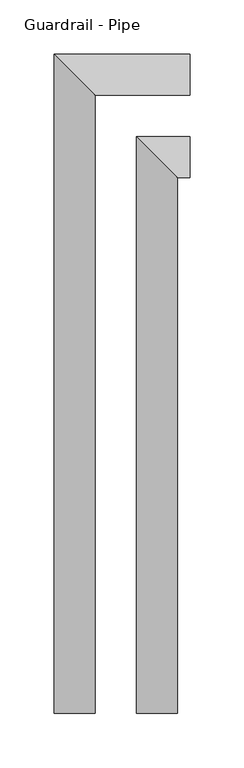
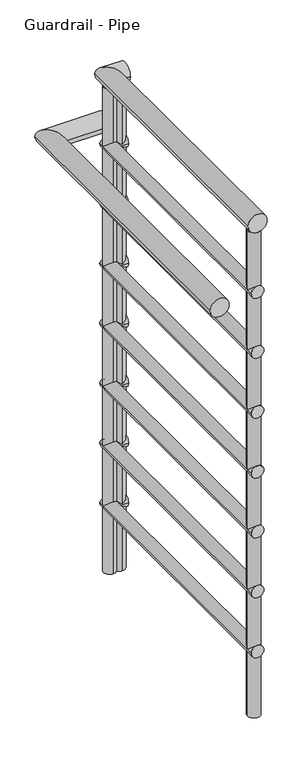
"""IFC4 building model written with IfcOpenShell, lengths in millimetres: railing geometry, Guardrail - Pipe."""

import ifcopenshell
import ifcopenshell.guid

model = None  # the IFC model being written
_history = None  # IfcOwnerHistory: only IFC2X3 demands one
_inside = {}  # id of a spatial element -> (the spatial element, [elements in it])
_under = {}  # id of a project, library or spatial element -> (it, [spatial elements below it])
_declared = {}  # id of a project -> (the project, [libraries it declares])
_typed = {}  # id of a type object -> (the type object, [elements of that type])
_made_of = {}  # id of a material, layer set ... -> (it, [elements and type objects made of it])


def new_model(schema):
    """Start an empty IFC model of exactly this schema.

    Asked for "IFC4X3", IfcOpenShell would pick the latest addendum, in which some entities
    have other attributes; the version numbers below select the first issue.
    IFC2X3 requires an IfcOwnerHistory on every rooted entity: one is made here for all.
    """
    global model, _history
    if schema == "IFC4X3":
        model = ifcopenshell.file(schema_version=(4, 3, 0, 0))
    else:
        model = ifcopenshell.file(schema=schema)
    _inside.clear()
    _under.clear()
    _declared.clear()
    _typed.clear()
    _made_of.clear()
    _history = None
    if model.schema == "IFC2X3":
        org = make("IfcOrganization", Name="unknown")
        user = make(
            "IfcPersonAndOrganization",
            ThePerson=make("IfcPerson", FamilyName="unknown"),
            TheOrganization=org,
        )
        app = make(
            "IfcApplication",
            ApplicationDeveloper=org,
            Version="unknown",
            ApplicationFullName="unknown",
            ApplicationIdentifier="unknown",
        )
        _history = make(
            "IfcOwnerHistory",
            OwningUser=user,
            OwningApplication=app,
            ChangeAction="ADDED",
            CreationDate=0,
        )
    return model


def make(cls, **values):
    """One entity of the class cls with the attributes given. An attribute that is None is left unset."""
    return model.create_entity(
        cls, **{name: value for name, value in values.items() if value is not None}
    )


def rooted(cls, **values):
    """An entity with a GlobalId (a new one), such as an element, a storey or a relation."""
    return make(cls, GlobalId=ifcopenshell.guid.new(), OwnerHistory=_history, **values)


def si_unit(unit_type, name, prefix=None):
    """IfcSIUnit, for example si_unit("LENGTHUNIT", "METRE", prefix="MILLI")."""
    return make("IfcSIUnit", UnitType=unit_type, Prefix=prefix, Name=name)


def assignment(units):
    """IfcUnitAssignment: the units of a project."""
    return None if units is None else make("IfcUnitAssignment", Units=units)


def point(xyz):
    """IfcCartesianPoint."""
    return None if xyz is None else make("IfcCartesianPoint", Coordinates=xyz)


def direction(xyz):
    """IfcDirection."""
    return None if xyz is None else make("IfcDirection", DirectionRatios=xyz)


def frame(location, z_axis=None, x_axis=None):
    """IfcAxis2Placement3D, a coordinate frame: its origin and axes. An axis left out is left unset."""
    return make(
        "IfcAxis2Placement3D",
        Location=point(location),
        Axis=direction(z_axis),
        RefDirection=direction(x_axis),
    )


def frame_2d(location, x_axis=None):
    """IfcAxis2Placement2D, a coordinate frame in the plane: its origin and x axis."""
    return make(
        "IfcAxis2Placement2D", Location=point(location), RefDirection=direction(x_axis)
    )


def origin():
    """The frame at (0, 0, 0) with its axes left unset."""
    return frame((0.0, 0.0, 0.0))


def place(relative_to, where):
    """IfcLocalPlacement: puts the frame where relative to a parent placement (None: the world)."""
    return make(
        "IfcLocalPlacement", PlacementRelTo=relative_to, RelativePlacement=where
    )


def context(
    kind, dimensions, precision=None, world=None, true_north=None, identifier=None
):
    """IfcGeometricRepresentationContext, for example the 3D "Model" context."""
    return make(
        "IfcGeometricRepresentationContext",
        ContextIdentifier=identifier,
        ContextType=kind,
        CoordinateSpaceDimension=dimensions,
        Precision=precision,
        WorldCoordinateSystem=world,
        TrueNorth=true_north,
    )


def project(units=None, contexts=None):
    """IfcProject with its units and contexts."""
    return rooted(
        "IfcProject",
        Name="project",
        RepresentationContexts=contexts,
        UnitsInContext=assignment(units),
    )


def spatial(cls, under=None, at=None, **own):
    """A site, building, storey or space (cls), placed at a placement, below another one or the project."""
    s = rooted(cls, ObjectPlacement=at, **own)
    if under is not None:
        _under.setdefault(under.id(), (under, []))[1].append(s)
    return s


def circle_curve(where, radius):
    """IfcCircle in the frame where."""
    return make("IfcCircle", Position=where, Radius=radius)


def ellipse_curve(where, semi_axis1, semi_axis2):
    """IfcEllipse in the frame where."""
    return make(
        "IfcEllipse", Position=where, SemiAxis1=semi_axis1, SemiAxis2=semi_axis2
    )


def trimmed(basis, trim1, trim2, sense, master):
    """IfcTrimmedCurve: the piece of a basis curve between two trims."""
    return make(
        "IfcTrimmedCurve",
        BasisCurve=basis,
        Trim1=trim1,
        Trim2=trim2,
        SenseAgreement=sense,
        MasterRepresentation=master,
    )


def segment(curve, same_sense, transition):
    """IfcCompositeCurveSegment."""
    return make(
        "IfcCompositeCurveSegment",
        Transition=transition,
        SameSense=same_sense,
        ParentCurve=curve,
    )


def composite_curve(segments, self_intersect=None):
    """IfcCompositeCurve: segments joined end to end."""
    return make("IfcCompositeCurve", Segments=segments, SelfIntersect=self_intersect)


def outline(outer, holes=None, kind="AREA"):
    """IfcArbitraryClosedProfileDef: a profile drawn as a closed curve; with holes, ...WithVoids."""
    if holes is None:
        return make("IfcArbitraryClosedProfileDef", ProfileType=kind, OuterCurve=outer)
    return make(
        "IfcArbitraryProfileDefWithVoids",
        ProfileType=kind,
        OuterCurve=outer,
        InnerCurves=holes,
    )


def extrude(swept, where, along, depth):
    """IfcExtrudedAreaSolid: the profile swept, set in the frame where, extruded along a direction by depth."""
    return make(
        "IfcExtrudedAreaSolid",
        SweptArea=swept,
        Position=where,
        ExtrudedDirection=direction(along),
        Depth=depth,
    )


def shape(context_of_items, identifier, shape_type, items):
    """IfcShapeRepresentation: the items that make up one representation, for example the "Body"."""
    return make(
        "IfcShapeRepresentation",
        ContextOfItems=context_of_items,
        RepresentationIdentifier=identifier,
        RepresentationType=shape_type,
        Items=items,
    )


def source(mapping_origin, context_of_items, identifier, shape_type, items):
    """IfcRepresentationMap: a shape defined once, which mapped items show again and again."""
    return make(
        "IfcRepresentationMap",
        MappingOrigin=mapping_origin,
        MappedRepresentation=shape(context_of_items, identifier, shape_type, items),
    )


def transform(
    local_origin,
    x_axis=None,
    y_axis=None,
    z_axis=None,
    scale=None,
    scale2=None,
    scale3=None,
    uniform=True,
):
    """IfcCartesianTransformationOperator3D, or its non-uniform kind. x_axis, y_axis, z_axis: its Axis1, 2, 3."""
    if uniform:
        return make(
            "IfcCartesianTransformationOperator3D",
            Axis1=direction(x_axis),
            Axis2=direction(y_axis),
            LocalOrigin=point(local_origin),
            Scale=scale,
            Axis3=direction(z_axis),
        )
    return make(
        "IfcCartesianTransformationOperator3DnonUniform",
        Axis1=direction(x_axis),
        Axis2=direction(y_axis),
        LocalOrigin=point(local_origin),
        Scale=scale,
        Axis3=direction(z_axis),
        Scale2=scale2,
        Scale3=scale3,
    )


def mapped(mapping_source, mapping_target):
    """IfcMappedItem: shows the shape of a source again, moved by a transform."""
    return make(
        "IfcMappedItem", MappingSource=mapping_source, MappingTarget=mapping_target
    )


def made_of(thing, what):
    """Note that an element or type object is made of a material, layer set ...; save() writes the relation."""
    if what is not None:
        _made_of.setdefault(what.id(), (what, []))[1].append(thing)
    return thing


def element(
    cls,
    number,
    at=None,
    inside=None,
    cuts=None,
    type_object=None,
    material=None,
    context=None,
    identifier="Body",
    shape_type=None,
    held_by="IfcProductDefinitionShape",
    body=None,
    shapes=None,
    **own,
):
    """One element of the class cls, such as IfcWall. Its Tag is "e" and its number.

    at: its placement. inside: the storey or other place that contains it. cuts: it is an
    opening in that element (IfcRelVoidsElement). A single representation is given by context,
    identifier, shape_type and body (its items); several are given by shapes. held_by: the class
    of the entity that holds the representations. save() writes the other relations.
    """
    e = rooted(cls, Tag="e%d" % number, ObjectPlacement=at, **own)
    if body is not None:
        shapes = [shape(context, identifier, shape_type, body)]
    if shapes is not None:
        e.Representation = make(held_by, Representations=shapes)
    if inside is not None:
        _inside.setdefault(inside.id(), (inside, []))[1].append(e)
    if cuts is not None:
        rooted(
            "IfcRelVoidsElement", RelatingBuildingElement=cuts, RelatedOpeningElement=e
        )
    if type_object is not None:
        _typed.setdefault(type_object.id(), (type_object, []))[1].append(e)
    return made_of(e, material)


def aggregate(whole, parts):
    """IfcRelAggregates: a whole, such as a stair, and the parts it consists of."""
    return rooted("IfcRelAggregates", RelatingObject=whole, RelatedObjects=parts)


def save(model, path):
    """Write the relations noted so far, then the file.

    IfcRelAggregates (storeys below a building ...), IfcRelContainedInSpatialStructure (elements
    in a storey), IfcRelDefinesByType, IfcRelAssociatesMaterial and IfcRelDeclares: one each for
    every whole, place, type object, material and project.
    """
    for whole, parts in _under.values():
        aggregate(whole, parts)
    for where, things in _inside.values():
        rooted(
            "IfcRelContainedInSpatialStructure",
            RelatedElements=things,
            RelatingStructure=where,
        )
    for kind, things in _typed.values():
        rooted("IfcRelDefinesByType", RelatedObjects=things, RelatingType=kind)
    for what, things in _made_of.values():
        rooted("IfcRelAssociatesMaterial", RelatedObjects=things, RelatingMaterial=what)
    for by, libraries in _declared.values():
        rooted("IfcRelDeclares", RelatingContext=by, RelatedDefinitions=libraries)
    model.write(path)


def plane_surface(at):
    """IfcPlane: the flat surface through the origin of the frame at, square to its z axis."""
    return make("IfcPlane", Position=at)


def cylinder_surface(at, radius):
    """IfcCylindricalSurface: all points at the distance radius from the z axis of the frame at."""
    return make("IfcCylindricalSurface", Position=at, Radius=radius)


def advanced_brep(points, edges, surfaces, faces):
    """IfcAdvancedBrep: a solid bounded by faces that lie on surfaces and meet in shared edges.

    An edge is (start, end): straight between two places in points (the first is 0);
    or (start, end, curve); or (start, end, curve, False) where it runs against its curve.
    A face is (place in surfaces, loops), or (place, loops, False) where it looks against
    its surface's normal. A loop lists edges by number (the first is 1), with a minus sign
    where the edge is run from its end to its start. The first loop is the outer one.
    """
    corners = [point(p) for p in points]
    vertices = [make("IfcVertexPoint", VertexGeometry=c) for c in corners]
    made = []
    for start, end, *more in edges:
        made.append(
            make(
                "IfcEdgeCurve",
                EdgeStart=vertices[start],
                EdgeEnd=vertices[end],
                EdgeGeometry=more[0] if more else make("IfcPolyline", Points=[corners[start], corners[end]]),
                SameSense=more[1] if len(more) > 1 else True,
            )
        )
    hull = []
    for where, loops, *sense in faces:
        bounds = []
        for j, loop in enumerate(loops):
            ring = [make("IfcOrientedEdge", EdgeElement=made[abs(k) - 1], Orientation=k > 0) for k in loop]
            bounds.append(
                make(
                    "IfcFaceOuterBound" if j == 0 else "IfcFaceBound",
                    Bound=make("IfcEdgeLoop", EdgeList=ring),
                    Orientation=True,
                )
            )
        hull.append(make("IfcAdvancedFace", Bounds=bounds, FaceSurface=surfaces[where], SameSense=sense[0] if sense else True))
    return make("IfcAdvancedBrep", Outer=make("IfcClosedShell", CfsFaces=hull))


def guardrail_pipe_cdf6dc9d(model_context):
    return source(origin(), model_context, "Body", "SolidModel", [
        advanced_brep(
        [(-10694.8293787, -5457.4797826, 4705.35), (-10656.7293787, -5457.4797826, 4705.35), (-10694.8293787, -4924.0797826, 4705.35), (-10656.7293787, -4962.1797826, 4705.35), (-10645.1029016, -4924.0797826, 4705.35), (-10645.1029016, -4962.1797826, 4705.35)],
        [
            (0, 1, circle_curve(frame((-10675.7793787, -5457.4797826, 4705.35), z_axis=(0.0, -1.0, 0.0), x_axis=(1.0, 0.0, 0.0)), 19.05)),
            (1, 0, circle_curve(frame((-10675.7793787, -5457.4797826, 4705.35), z_axis=(0.0, -1.0, 0.0), x_axis=(1.0, 0.0, 0.0)), 19.05)),
            (2, 3, ellipse_curve(frame((-10675.7793787, -4943.1297826, 4705.35), z_axis=(-0.7071067811865502, -0.7071067811865449, 0.0), x_axis=(-0.707106781186545, 0.70710678118655, 0.0)), 26.9407684, 19.05)),
            (3, 1),
            (0, 2),
            (3, 2, ellipse_curve(frame((-10675.7793787, -4943.1297826, 4705.35), z_axis=(-0.7071067811865502, -0.7071067811865449, 0.0), x_axis=(-0.707106781186545, 0.70710678118655, 0.0)), 26.9407684, 19.05)),
            (4, 5, circle_curve(frame((-10645.1029016, -4943.1297826, 4705.35), z_axis=(1.0, 0.0, 0.0), x_axis=(0.0, -1.0, 0.0)), 19.05)),
            (5, 4, circle_curve(frame((-10645.1029016, -4943.1297826, 4705.35), z_axis=(1.0, 0.0, 0.0), x_axis=(0.0, -1.0, 0.0)), 19.05)),
            (5, 3),
            (2, 4),
        ],
        [
            plane_surface(frame((-10675.7793787, -5457.4797826, 4724.4), z_axis=(0.0, -1.0, 0.0), x_axis=(0.0, 0.0, -1.0))),
            cylinder_surface(frame((-10675.7793787, -4943.1297826, 4705.35), z_axis=(0.0, 1.0, 0.0), x_axis=(1.0, 0.0, 0.0)), 19.05),
            plane_surface(frame((-10645.1029016, -4943.1297826, 4724.4), z_axis=(1.0, 0.0, 0.0), x_axis=(0.0, -1.0, 0.0))),
            cylinder_surface(frame((-10645.1029016, -4943.1297826, 4705.35), z_axis=(1.0, 0.0, 0.0), x_axis=(0.0, -1.0, 0.0)), 19.05),
        ],
        [
            (0, [[1, 2]]),
            (1, [[3, 4, -1, 5]]),
            (1, [[6, -5, -2, -4]]),
            (2, [[7, 8]]),
            (3, [[-8, 9, -3, 10]]),
            (3, [[-7, -10, -6, -9]]),
        ],
    ),
        advanced_brep(
        [(-10645.1029016, -4930.4297826, 4559.3), (-10645.1029016, -4955.8297826, 4559.3), (-10663.0793787, -4955.8297826, 4559.3), (-10688.4793787, -4930.4297826, 4559.3), (-10688.4793787, -5457.4797826, 4559.3), (-10663.0793787, -5457.4797826, 4559.3)],
        [
            (0, 1, circle_curve(frame((-10645.1029016, -4943.1297826, 4559.3), z_axis=(1.0, 0.0, 0.0), x_axis=(0.0, -1.0, 0.0)), 12.7)),
            (1, 0, circle_curve(frame((-10645.1029016, -4943.1297826, 4559.3), z_axis=(1.0, 0.0, 0.0), x_axis=(0.0, -1.0, 0.0)), 12.7)),
            (1, 2),
            (2, 3, ellipse_curve(frame((-10675.7793787, -4943.1297826, 4559.3), z_axis=(0.7071067811865502, 0.7071067811865449, 0.0), x_axis=(0.7071067811865447, -0.7071067811865503, 0.0)), 17.9605122, 12.7)),
            (3, 0),
            (3, 2, ellipse_curve(frame((-10675.7793787, -4943.1297826, 4559.3), z_axis=(0.7071067811865502, 0.7071067811865449, 0.0), x_axis=(0.7071067811865447, -0.7071067811865503, 0.0)), 17.9605122, 12.7)),
            (4, 5, circle_curve(frame((-10675.7793787, -5457.4797826, 4559.3), z_axis=(0.0, -1.0, 0.0), x_axis=(1.0, 0.0, 0.0)), 12.7)),
            (5, 4, circle_curve(frame((-10675.7793787, -5457.4797826, 4559.3), z_axis=(0.0, -1.0, 0.0), x_axis=(1.0, 0.0, 0.0)), 12.7)),
            (2, 5),
            (4, 3),
        ],
        [
            plane_surface(frame((-10645.1029016, -4943.1297826, 4572.0), z_axis=(1.0, 0.0, 0.0), x_axis=(0.0, -1.0, 0.0))),
            cylinder_surface(frame((-10645.1029016, -4943.1297826, 4559.3), z_axis=(1.0, 0.0, 0.0), x_axis=(0.0, -1.0, 0.0)), 12.7),
            plane_surface(frame((-10675.7793787, -5457.4797826, 4572.0), z_axis=(0.0, -1.0, 0.0), x_axis=(0.0, 0.0, -1.0))),
            cylinder_surface(frame((-10675.7793787, -4943.1297826, 4559.3), z_axis=(0.0, 1.0, 0.0), x_axis=(1.0, 0.0, 0.0)), 12.7),
        ],
        [
            (0, [[1, 2]]),
            (1, [[-2, 3, 4, 5]]),
            (1, [[-1, -5, 6, -3]]),
            (2, [[7, 8]]),
            (3, [[-4, 9, -7, 10]]),
            (3, [[-6, -10, -8, -9]]),
        ],
    ),
        advanced_brep(
        [(-10771.0293787, -5457.4797826, 4552.95), (-10732.9293787, -5457.4797826, 4552.95), (-10771.0293787, -4847.8797826, 4552.95), (-10732.9293787, -4885.9797826, 4552.95), (-10645.1029016, -4847.8797826, 4552.95), (-10645.1029016, -4885.9797826, 4552.95)],
        [
            (0, 1, circle_curve(frame((-10751.9793787, -5457.4797826, 4552.95), z_axis=(0.0, -1.0, 0.0), x_axis=(1.0, 0.0, 0.0)), 19.05)),
            (1, 0, circle_curve(frame((-10751.9793787, -5457.4797826, 4552.95), z_axis=(0.0, -1.0, 0.0), x_axis=(1.0, 0.0, 0.0)), 19.05)),
            (2, 3, ellipse_curve(frame((-10751.9793787, -4866.9297826, 4552.95), z_axis=(-0.7071067811865502, -0.7071067811865449, 0.0), x_axis=(-0.707106781186545, 0.70710678118655, 0.0)), 26.9407684, 19.05)),
            (3, 1),
            (0, 2),
            (3, 2, ellipse_curve(frame((-10751.9793787, -4866.9297826, 4552.95), z_axis=(-0.7071067811865502, -0.7071067811865449, 0.0), x_axis=(-0.707106781186545, 0.70710678118655, 0.0)), 26.9407684, 19.05)),
            (4, 5, circle_curve(frame((-10645.1029016, -4866.9297826, 4552.95), z_axis=(1.0, 0.0, 0.0), x_axis=(0.0, -1.0, 0.0)), 19.05)),
            (5, 4, circle_curve(frame((-10645.1029016, -4866.9297826, 4552.95), z_axis=(1.0, 0.0, 0.0), x_axis=(0.0, -1.0, 0.0)), 19.05)),
            (4, 2),
            (3, 5),
        ],
        [
            plane_surface(frame((-10751.9793787, -5457.4797826, 4572.0), z_axis=(0.0, -1.0, 0.0), x_axis=(0.0, 0.0, -1.0))),
            cylinder_surface(frame((-10751.9793787, -4866.9297826, 4552.95), z_axis=(0.0, 1.0, 0.0), x_axis=(1.0, 0.0, 0.0)), 19.05),
            plane_surface(frame((-10645.1029016, -4866.9297826, 4572.0), z_axis=(1.0, 0.0, 0.0), x_axis=(0.0, -1.0, 0.0))),
            cylinder_surface(frame((-10645.1029016, -4866.9297826, 4552.95), z_axis=(1.0, 0.0, 0.0), x_axis=(0.0, -1.0, 0.0)), 19.05),
        ],
        [
            (0, [[1, 2]]),
            (1, [[3, 4, -1, 5]]),
            (1, [[6, -5, -2, -4]]),
            (2, [[7, 8]]),
            (3, [[-7, 9, -6, 10]]),
            (3, [[-8, -10, -3, -9]]),
        ],
    ),
        advanced_brep(
        [(-10645.1029016, -4930.4297826, 4432.3), (-10645.1029016, -4955.8297826, 4432.3), (-10663.0793787, -4955.8297826, 4432.3), (-10688.4793787, -4930.4297826, 4432.3), (-10688.4793787, -5457.4797826, 4432.3), (-10663.0793787, -5457.4797826, 4432.3)],
        [
            (0, 1, circle_curve(frame((-10645.1029016, -4943.1297826, 4432.3), z_axis=(1.0, 0.0, 0.0), x_axis=(0.0, -1.0, 0.0)), 12.7)),
            (1, 0, circle_curve(frame((-10645.1029016, -4943.1297826, 4432.3), z_axis=(1.0, 0.0, 0.0), x_axis=(0.0, -1.0, 0.0)), 12.7)),
            (1, 2),
            (2, 3, ellipse_curve(frame((-10675.7793787, -4943.1297826, 4432.3), z_axis=(0.7071067811865502, 0.7071067811865449, 0.0), x_axis=(0.7071067811865447, -0.7071067811865503, 0.0)), 17.9605122, 12.7)),
            (3, 0),
            (3, 2, ellipse_curve(frame((-10675.7793787, -4943.1297826, 4432.3), z_axis=(0.7071067811865502, 0.7071067811865449, 0.0), x_axis=(0.7071067811865447, -0.7071067811865503, 0.0)), 17.9605122, 12.7)),
            (4, 5, circle_curve(frame((-10675.7793787, -5457.4797826, 4432.3), z_axis=(0.0, -1.0, 0.0), x_axis=(1.0, 0.0, 0.0)), 12.7)),
            (5, 4, circle_curve(frame((-10675.7793787, -5457.4797826, 4432.3), z_axis=(0.0, -1.0, 0.0), x_axis=(1.0, 0.0, 0.0)), 12.7)),
            (2, 5),
            (4, 3),
        ],
        [
            plane_surface(frame((-10645.1029016, -4943.1297826, 4445.0), z_axis=(1.0, 0.0, 0.0), x_axis=(0.0, -1.0, 0.0))),
            cylinder_surface(frame((-10645.1029016, -4943.1297826, 4432.3), z_axis=(1.0, 0.0, 0.0), x_axis=(0.0, -1.0, 0.0)), 12.7),
            plane_surface(frame((-10675.7793787, -5457.4797826, 4445.0), z_axis=(0.0, -1.0, 0.0), x_axis=(0.0, 0.0, -1.0))),
            cylinder_surface(frame((-10675.7793787, -4943.1297826, 4432.3), z_axis=(0.0, 1.0, 0.0), x_axis=(1.0, 0.0, 0.0)), 12.7),
        ],
        [
            (0, [[1, 2]]),
            (1, [[-2, 3, 4, 5]]),
            (1, [[-1, -5, 6, -3]]),
            (2, [[7, 8]]),
            (3, [[-4, 9, -7, 10]]),
            (3, [[-6, -10, -8, -9]]),
        ],
    ),
        advanced_brep(
        [(-10645.1029016, -4930.4297826, 4305.3), (-10645.1029016, -4955.8297826, 4305.3), (-10663.0793787, -4955.8297826, 4305.3), (-10688.4793787, -4930.4297826, 4305.3), (-10688.4793787, -5457.4797826, 4305.3), (-10663.0793787, -5457.4797826, 4305.3)],
        [
            (0, 1, circle_curve(frame((-10645.1029016, -4943.1297826, 4305.3), z_axis=(1.0, 0.0, 0.0), x_axis=(0.0, -1.0, 0.0)), 12.7)),
            (1, 0, circle_curve(frame((-10645.1029016, -4943.1297826, 4305.3), z_axis=(1.0, 0.0, 0.0), x_axis=(0.0, -1.0, 0.0)), 12.7)),
            (1, 2),
            (2, 3, ellipse_curve(frame((-10675.7793787, -4943.1297826, 4305.3), z_axis=(0.7071067811865502, 0.7071067811865449, 0.0), x_axis=(0.7071067811865447, -0.7071067811865503, 0.0)), 17.9605122, 12.7)),
            (3, 0),
            (3, 2, ellipse_curve(frame((-10675.7793787, -4943.1297826, 4305.3), z_axis=(0.7071067811865502, 0.7071067811865449, 0.0), x_axis=(0.7071067811865447, -0.7071067811865503, 0.0)), 17.9605122, 12.7)),
            (4, 5, circle_curve(frame((-10675.7793787, -5457.4797826, 4305.3), z_axis=(0.0, -1.0, 0.0), x_axis=(1.0, 0.0, 0.0)), 12.7)),
            (5, 4, circle_curve(frame((-10675.7793787, -5457.4797826, 4305.3), z_axis=(0.0, -1.0, 0.0), x_axis=(1.0, 0.0, 0.0)), 12.7)),
            (2, 5),
            (4, 3),
        ],
        [
            plane_surface(frame((-10645.1029016, -4943.1297826, 4318.0), z_axis=(1.0, 0.0, 0.0), x_axis=(0.0, -1.0, 0.0))),
            cylinder_surface(frame((-10645.1029016, -4943.1297826, 4305.3), z_axis=(1.0, 0.0, 0.0), x_axis=(0.0, -1.0, 0.0)), 12.7),
            plane_surface(frame((-10675.7793787, -5457.4797826, 4318.0), z_axis=(0.0, -1.0, 0.0), x_axis=(0.0, 0.0, -1.0))),
            cylinder_surface(frame((-10675.7793787, -4943.1297826, 4305.3), z_axis=(0.0, 1.0, 0.0), x_axis=(1.0, 0.0, 0.0)), 12.7),
        ],
        [
            (0, [[1, 2]]),
            (1, [[-2, 3, 4, 5]]),
            (1, [[-1, -5, 6, -3]]),
            (2, [[7, 8]]),
            (3, [[-4, 9, -7, 10]]),
            (3, [[-6, -10, -8, -9]]),
        ],
    ),
        advanced_brep(
        [(-10645.1029016, -4930.4297826, 4178.3), (-10645.1029016, -4955.8297826, 4178.3), (-10663.0793787, -4955.8297826, 4178.3), (-10688.4793787, -4930.4297826, 4178.3), (-10688.4793787, -5457.4797826, 4178.3), (-10663.0793787, -5457.4797826, 4178.3)],
        [
            (0, 1, circle_curve(frame((-10645.1029016, -4943.1297826, 4178.3), z_axis=(1.0, 0.0, 0.0), x_axis=(0.0, -1.0, 0.0)), 12.7)),
            (1, 0, circle_curve(frame((-10645.1029016, -4943.1297826, 4178.3), z_axis=(1.0, 0.0, 0.0), x_axis=(0.0, -1.0, 0.0)), 12.7)),
            (1, 2),
            (2, 3, ellipse_curve(frame((-10675.7793787, -4943.1297826, 4178.3), z_axis=(0.7071067811865502, 0.7071067811865449, 0.0), x_axis=(0.7071067811865447, -0.7071067811865503, 0.0)), 17.9605122, 12.7)),
            (3, 0),
            (3, 2, ellipse_curve(frame((-10675.7793787, -4943.1297826, 4178.3), z_axis=(0.7071067811865502, 0.7071067811865449, 0.0), x_axis=(0.7071067811865447, -0.7071067811865503, 0.0)), 17.9605122, 12.7)),
            (4, 5, circle_curve(frame((-10675.7793787, -5457.4797826, 4178.3), z_axis=(0.0, -1.0, 0.0), x_axis=(1.0, 0.0, 0.0)), 12.7)),
            (5, 4, circle_curve(frame((-10675.7793787, -5457.4797826, 4178.3), z_axis=(0.0, -1.0, 0.0), x_axis=(1.0, 0.0, 0.0)), 12.7)),
            (2, 5),
            (4, 3),
        ],
        [
            plane_surface(frame((-10645.1029016, -4943.1297826, 4191.0), z_axis=(1.0, 0.0, 0.0), x_axis=(0.0, -1.0, 0.0))),
            cylinder_surface(frame((-10645.1029016, -4943.1297826, 4178.3), z_axis=(1.0, 0.0, 0.0), x_axis=(0.0, -1.0, 0.0)), 12.7),
            plane_surface(frame((-10675.7793787, -5457.4797826, 4191.0), z_axis=(0.0, -1.0, 0.0), x_axis=(0.0, 0.0, -1.0))),
            cylinder_surface(frame((-10675.7793787, -4943.1297826, 4178.3), z_axis=(0.0, 1.0, 0.0), x_axis=(1.0, 0.0, 0.0)), 12.7),
        ],
        [
            (0, [[1, 2]]),
            (1, [[-2, 3, 4, 5]]),
            (1, [[-1, -5, 6, -3]]),
            (2, [[7, 8]]),
            (3, [[-4, 9, -7, 10]]),
            (3, [[-6, -10, -8, -9]]),
        ],
    ),
        advanced_brep(
        [(-10645.1029016, -4930.4297826, 4051.3), (-10645.1029016, -4955.8297826, 4051.3), (-10663.0793787, -4955.8297826, 4051.3), (-10688.4793787, -4930.4297826, 4051.3), (-10688.4793787, -5457.4797826, 4051.3), (-10663.0793787, -5457.4797826, 4051.3)],
        [
            (0, 1, circle_curve(frame((-10645.1029016, -4943.1297826, 4051.3), z_axis=(1.0, 0.0, 0.0), x_axis=(0.0, -1.0, 0.0)), 12.7)),
            (1, 0, circle_curve(frame((-10645.1029016, -4943.1297826, 4051.3), z_axis=(1.0, 0.0, 0.0), x_axis=(0.0, -1.0, 0.0)), 12.7)),
            (1, 2),
            (2, 3, ellipse_curve(frame((-10675.7793787, -4943.1297826, 4051.3), z_axis=(0.7071067811865502, 0.7071067811865449, 0.0), x_axis=(0.7071067811865447, -0.7071067811865503, 0.0)), 17.9605122, 12.7)),
            (3, 0),
            (3, 2, ellipse_curve(frame((-10675.7793787, -4943.1297826, 4051.3), z_axis=(0.7071067811865502, 0.7071067811865449, 0.0), x_axis=(0.7071067811865447, -0.7071067811865503, 0.0)), 17.9605122, 12.7)),
            (4, 5, circle_curve(frame((-10675.7793787, -5457.4797826, 4051.3), z_axis=(0.0, -1.0, 0.0), x_axis=(1.0, 0.0, 0.0)), 12.7)),
            (5, 4, circle_curve(frame((-10675.7793787, -5457.4797826, 4051.3), z_axis=(0.0, -1.0, 0.0), x_axis=(1.0, 0.0, 0.0)), 12.7)),
            (2, 5),
            (4, 3),
        ],
        [
            plane_surface(frame((-10645.1029016, -4943.1297826, 4064.0), z_axis=(1.0, 0.0, 0.0), x_axis=(0.0, -1.0, 0.0))),
            cylinder_surface(frame((-10645.1029016, -4943.1297826, 4051.3), z_axis=(1.0, 0.0, 0.0), x_axis=(0.0, -1.0, 0.0)), 12.7),
            plane_surface(frame((-10675.7793787, -5457.4797826, 4064.0), z_axis=(0.0, -1.0, 0.0), x_axis=(0.0, 0.0, -1.0))),
            cylinder_surface(frame((-10675.7793787, -4943.1297826, 4051.3), z_axis=(0.0, 1.0, 0.0), x_axis=(1.0, 0.0, 0.0)), 12.7),
        ],
        [
            (0, [[1, 2]]),
            (1, [[-2, 3, 4, 5]]),
            (1, [[-1, -5, 6, -3]]),
            (2, [[7, 8]]),
            (3, [[-4, 9, -7, 10]]),
            (3, [[-6, -10, -8, -9]]),
        ],
    ),
        advanced_brep(
        [(-10645.1029016, -4930.4297826, 3924.3), (-10645.1029016, -4955.8297826, 3924.3), (-10663.0793787, -4955.8297826, 3924.3), (-10688.4793787, -4930.4297826, 3924.3), (-10688.4793787, -5457.4797826, 3924.3), (-10663.0793787, -5457.4797826, 3924.3)],
        [
            (0, 1, circle_curve(frame((-10645.1029016, -4943.1297826, 3924.3), z_axis=(1.0, 0.0, 0.0), x_axis=(0.0, -1.0, 0.0)), 12.7)),
            (1, 0, circle_curve(frame((-10645.1029016, -4943.1297826, 3924.3), z_axis=(1.0, 0.0, 0.0), x_axis=(0.0, -1.0, 0.0)), 12.7)),
            (1, 2),
            (2, 3, ellipse_curve(frame((-10675.7793787, -4943.1297826, 3924.3), z_axis=(0.7071067811865502, 0.7071067811865449, 0.0), x_axis=(0.7071067811865447, -0.7071067811865503, 0.0)), 17.9605122, 12.7)),
            (3, 0),
            (3, 2, ellipse_curve(frame((-10675.7793787, -4943.1297826, 3924.3), z_axis=(0.7071067811865502, 0.7071067811865449, 0.0), x_axis=(0.7071067811865447, -0.7071067811865503, 0.0)), 17.9605122, 12.7)),
            (4, 5, circle_curve(frame((-10675.7793787, -5457.4797826, 3924.3), z_axis=(0.0, -1.0, 0.0), x_axis=(1.0, 0.0, 0.0)), 12.7)),
            (5, 4, circle_curve(frame((-10675.7793787, -5457.4797826, 3924.3), z_axis=(0.0, -1.0, 0.0), x_axis=(1.0, 0.0, 0.0)), 12.7)),
            (2, 5),
            (4, 3),
        ],
        [
            plane_surface(frame((-10645.1029016, -4943.1297826, 3937.0), z_axis=(1.0, 0.0, 0.0), x_axis=(0.0, -1.0, 0.0))),
            cylinder_surface(frame((-10645.1029016, -4943.1297826, 3924.3), z_axis=(1.0, 0.0, 0.0), x_axis=(0.0, -1.0, 0.0)), 12.7),
            plane_surface(frame((-10675.7793787, -5457.4797826, 3937.0), z_axis=(0.0, -1.0, 0.0), x_axis=(0.0, 0.0, -1.0))),
            cylinder_surface(frame((-10675.7793787, -4943.1297826, 3924.3), z_axis=(0.0, 1.0, 0.0), x_axis=(1.0, 0.0, 0.0)), 12.7),
        ],
        [
            (0, [[1, 2]]),
            (1, [[-2, 3, 4, 5]]),
            (1, [[-1, -5, 6, -3]]),
            (2, [[7, 8]]),
            (3, [[-4, 9, -7, 10]]),
            (3, [[-6, -10, -8, -9]]),
        ],
    ),
        advanced_brep(
        [(-10645.1029016, -4930.4297826, 3797.3), (-10645.1029016, -4955.8297826, 3797.3), (-10663.0793787, -4955.8297826, 3797.3), (-10688.4793787, -4930.4297826, 3797.3), (-10688.4793787, -5457.4797826, 3797.3), (-10663.0793787, -5457.4797826, 3797.3)],
        [
            (0, 1, circle_curve(frame((-10645.1029016, -4943.1297826, 3797.3), z_axis=(1.0, 0.0, 0.0), x_axis=(0.0, -1.0, 0.0)), 12.7)),
            (1, 0, circle_curve(frame((-10645.1029016, -4943.1297826, 3797.3), z_axis=(1.0, 0.0, 0.0), x_axis=(0.0, -1.0, 0.0)), 12.7)),
            (1, 2),
            (2, 3, ellipse_curve(frame((-10675.7793787, -4943.1297826, 3797.3), z_axis=(0.7071067811865502, 0.7071067811865449, 0.0), x_axis=(0.7071067811865447, -0.7071067811865503, 0.0)), 17.9605122, 12.7)),
            (3, 0),
            (3, 2, ellipse_curve(frame((-10675.7793787, -4943.1297826, 3797.3), z_axis=(0.7071067811865502, 0.7071067811865449, 0.0), x_axis=(0.7071067811865447, -0.7071067811865503, 0.0)), 17.9605122, 12.7)),
            (4, 5, circle_curve(frame((-10675.7793787, -5457.4797826, 3797.3), z_axis=(0.0, -1.0, 0.0), x_axis=(1.0, 0.0, 0.0)), 12.7)),
            (5, 4, circle_curve(frame((-10675.7793787, -5457.4797826, 3797.3), z_axis=(0.0, -1.0, 0.0), x_axis=(1.0, 0.0, 0.0)), 12.7)),
            (2, 5),
            (4, 3),
        ],
        [
            plane_surface(frame((-10645.1029016, -4943.1297826, 3810.0), z_axis=(1.0, 0.0, 0.0), x_axis=(0.0, -1.0, 0.0))),
            cylinder_surface(frame((-10645.1029016, -4943.1297826, 3797.3), z_axis=(1.0, 0.0, 0.0), x_axis=(0.0, -1.0, 0.0)), 12.7),
            plane_surface(frame((-10675.7793787, -5457.4797826, 3810.0), z_axis=(0.0, -1.0, 0.0), x_axis=(0.0, 0.0, -1.0))),
            cylinder_surface(frame((-10675.7793787, -4943.1297826, 3797.3), z_axis=(0.0, 1.0, 0.0), x_axis=(1.0, 0.0, 0.0)), 12.7),
        ],
        [
            (0, [[1, 2]]),
            (1, [[-2, 3, 4, 5]]),
            (1, [[-1, -5, 6, -3]]),
            (2, [[7, 8]]),
            (3, [[-4, 9, -7, 10]]),
            (3, [[-6, -10, -8, -9]]),
        ],
    ),
        extrude(outline(composite_curve([segment(trimmed(circle_curve(frame_2d((-10675.7793787, -4943.1297826)), 12.7), [point((-10675.7793787, -4930.4297826))], [point((-10675.7793787, -4955.8297826))], False, "CARTESIAN"), True, "CONTINUOUS"), segment(trimmed(circle_curve(frame_2d((-10675.7793787, -4943.1297826)), 12.7), [point((-10675.7793787, -4955.8297826))], [point((-10675.7793787, -4930.4297826))], False, "CARTESIAN"), True, "CONTINUOUS")], self_intersect=False)), frame((0.0, 0.0, 3657.6), z_axis=(0.0, 0.0, 1.0), x_axis=(1.0, 0.0, 0.0)), (0.0, 0.0, 1.0), 1028.7),
        extrude(outline(composite_curve([segment(trimmed(circle_curve(frame_2d((-10675.7793787, -5444.7797826)), 12.7), [point((-10688.4793787, -5444.7797826))], [point((-10663.0793787, -5444.7797826))], False, "CARTESIAN"), True, "CONTINUOUS"), segment(trimmed(circle_curve(frame_2d((-10675.7793787, -5444.7797826)), 12.7), [point((-10663.0793787, -5444.7797826))], [point((-10688.4793787, -5444.7797826))], False, "CARTESIAN"), True, "CONTINUOUS")], self_intersect=False)), frame((0.0, 0.0, 3657.6), z_axis=(0.0, 0.0, 1.0), x_axis=(1.0, 0.0, 0.0)), (0.0, 0.0, 1.0), 1028.7),
        extrude(outline(composite_curve([segment(trimmed(circle_curve(frame_2d((-10657.8029016, -4943.1297826)), 12.7), [point((-10657.8029016, -4930.4297826))], [point((-10657.8029016, -4955.8297826))], False, "CARTESIAN"), True, "CONTINUOUS"), segment(trimmed(circle_curve(frame_2d((-10657.8029016, -4943.1297826)), 12.7), [point((-10657.8029016, -4955.8297826))], [point((-10657.8029016, -4930.4297826))], False, "CARTESIAN"), True, "CONTINUOUS")], self_intersect=False)), frame((0.0, 0.0, 3657.6), z_axis=(0.0, 0.0, 1.0), x_axis=(1.0, 0.0, 0.0)), (0.0, 0.0, 1.0), 1028.7),
    ])


if __name__ == "__main__":
    model = new_model("IFC4")
    model_context = context("Model", 3, world=origin())
    ifc_project = project(units=[si_unit("LENGTHUNIT", "METRE", prefix="MILLI")], contexts=[model_context])
    site = spatial("IfcSite", under=ifc_project)
    building = spatial("IfcBuilding", under=site)
    placement = place(None, origin())
    guardrail_pipe_shape = guardrail_pipe_cdf6dc9d(model_context)
    element("IfcRailing", 1, ObjectType="Guardrail - Pipe", at=placement, inside=building, context=model_context, shape_type="MappedRepresentation", body=[
        mapped(guardrail_pipe_shape, transform((0.0, 0.0, 0.0), x_axis=(1.0, 0.0, 0.0), y_axis=(0.0, 1.0, 0.0), z_axis=(0.0, 0.0, 1.0))),
    ])
    save(model, "model.ifc")

# Revit data of these elements
# Element 1 (IfcRailing, "Guardrail - Pipe")
#   Materials on its faces: "Plastic - Vinyl Cove Base"
# Materials
#   "Plastic - Vinyl Cove Base": class "Plastic", colour RGB 5 5 5, transparency 0, Cost = 0
